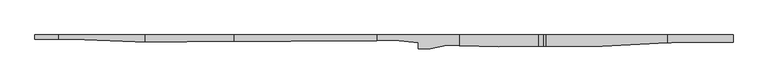
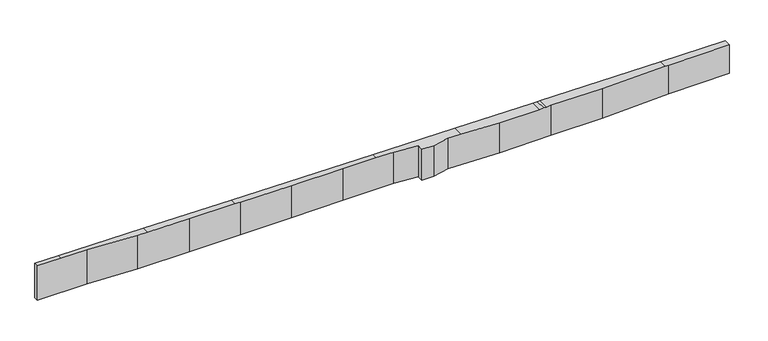
"""IFC4 building model written with IfcOpenShell, lengths in millimetres: proxy geometry, Flowable Fill : Flowable Fill."""

from ifc_helpers import new_model, si_unit, origin, place, context, project, spatial, faceted_brep, source, transform, mapped, element, save


def generic_models_da6e01de(model_context):
    return source(origin(), model_context, "Body", "Brep", [
        faceted_brep([(-76504.8, -1168.4, 8756.65), (-76504.8, -685.8, 8756.65), (0.0, -685.8, 8756.65), (0.0, -1498.6, 8756.65), (-6756.4, -1549.4, 8756.65), (-14325.6, -1905.0, 8756.65), (-20015.2, -1905.0, 8756.65), (-25704.8, -1981.2, 8756.65), (-31394.4, -1828.8, 8756.65), (-33197.8, -2224.0875, 8756.65), (-34493.2, -2224.0875, 8756.65), (-34493.2, -1538.2875, 8756.65), (-37084.0, -1295.4, 8756.65), (-42773.6, -1320.8, 8756.65), (-48463.2, -1371.6, 8756.65), (-54152.8, -1371.6, 8756.65), (-59842.4, -1447.8, 8756.65), (-65532.0, -1447.8, 8756.65), (-71018.4, -1193.8, 8756.65), (-71018.4, -1193.8, 12752.9363716), (-73924.5154607, -1180.3457618, 12775.8590028), (-76504.8, -1168.4, 12775.8590028), (-65532.0, -1447.8, 12709.661173), (-59842.4, -1447.8, 12630.8044454), (-64486.32492, -1447.8, 12701.4131786), (-54152.8, -1371.6, 12547.5273927), (-54739.2258845, -1379.4539181, 12553.2130404), (-48463.2, -1371.6, 12492.3643078), (-42773.6, -1320.8, 12437.2012228), (-37084.0, -1295.4, 12386.3772486), (-39060.1554467, -1304.2221225, 12401.197803), (-25704.8, -1981.2, 12287.5909977), (-29992.6104464, -1866.3479345, 12333.1940212), (-31394.4, -1828.8, 12343.7070091), (-20015.2, -1905.0, 12254.2742414), (-20545.0629958, -1912.0963794, 12259.7009275), (-20822.3850062, -1915.8105135, 12258.8865049), (-21332.1380629, -1922.6375633, 12241.0855359), (-14325.6, -1905.0, 12196.0031916), (-6756.4, -1549.4, 12121.4878946), (-7146.1405773, -1567.70996, 12122.4734818), (0.0, -1498.6, 12104.4021161), (0.0, -685.8, 12104.4021161), (-76504.8, -685.8, 12775.8590028), (-73924.5154607, -685.8, 12775.8590028), (-64486.32492, -685.8, 12701.4131786), (-54739.2258845, -685.8, 12553.2130404), (-39060.1554467, -685.8, 12401.197803), (-29992.6104464, -685.8, 12333.1940212), (-21332.1380629, -685.8, 12241.0855359), (-20822.3850062, -685.8, 12258.8865049), (-20545.0629958, -685.8, 12259.7009275), (-7146.1405773, -685.8, 12122.4734818), (-34493.2, -1538.2875, 12366.9470503), (-34493.2, -2224.0875, 12366.9470503), (-33197.8, -2224.0875, 12357.2319511)], [[[0, 1, 2, 3, 4, 5, 6, 7, 8, 9, 10, 11, 12, 13, 14, 15, 16, 17, 18]], [[0, 18, 19, 20, 21]], [[18, 17, 22, 19]], [[17, 16, 23, 24, 22]], [[16, 15, 25, 26, 23]], [[15, 14, 27, 25]], [[14, 13, 28, 27]], [[13, 12, 29, 30, 28]], [[8, 7, 31, 32, 33]], [[7, 6, 34, 35, 36, 37, 31]], [[6, 5, 38, 34]], [[5, 4, 39, 40, 38]], [[4, 3, 41, 39]], [[3, 2, 42, 41]], [[2, 1, 43, 44, 45, 46, 47, 48, 49, 50, 51, 52, 42]], [[1, 0, 21, 43]], [[52, 40, 39, 41, 42]], [[20, 44, 43, 21]], [[44, 20, 19, 22, 24, 45]], [[45, 24, 23, 26, 46]], [[46, 26, 25, 27, 28, 30, 47]], [[47, 30, 29, 53, 54, 55, 33, 32, 48]], [[48, 32, 31, 37, 49]], [[49, 37, 36, 50]], [[50, 36, 35, 51]], [[40, 52, 51, 35, 34, 38]], [[12, 11, 53, 29]], [[11, 10, 54, 53]], [[10, 9, 55, 54]], [[9, 8, 33, 55]]]),
    ])


if __name__ == "__main__":
    model = new_model("IFC4")
    model_context = context("Model", 3, world=origin())
    ifc_project = project(units=[si_unit("LENGTHUNIT", "METRE", prefix="MILLI")], contexts=[model_context])
    site = spatial("IfcSite", under=ifc_project)
    building = spatial("IfcBuilding", under=site)
    placement = place(None, origin())
    generic_models_shape = generic_models_da6e01de(model_context)
    element("IfcBuildingElementProxy", 1, Name="Flowable Fill : Flowable Fill", ObjectType="Flowable Fill : Flowable Fill", at=placement, inside=building, context=model_context, shape_type="MappedRepresentation", body=[
        mapped(generic_models_shape, transform((0.0, 0.0, 0.0), x_axis=(1.0, 0.0, 0.0), y_axis=(0.0, 1.0, 0.0), z_axis=(0.0, 0.0, 1.0))),
    ])
    save(model, "model.ifc")

# Revit data of these elements
# Element 1 (IfcBuildingElementProxy, "Flowable Fill : Flowable Fill")
#   Materials on its faces: "Site - Flowable Fill"
# Materials
#   "Site - Flowable Fill": class "Generic", colour RGB 255 0 128, transparency 0, Cost = 0
